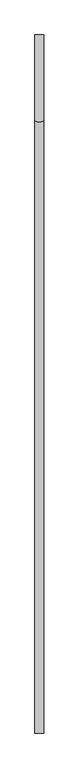
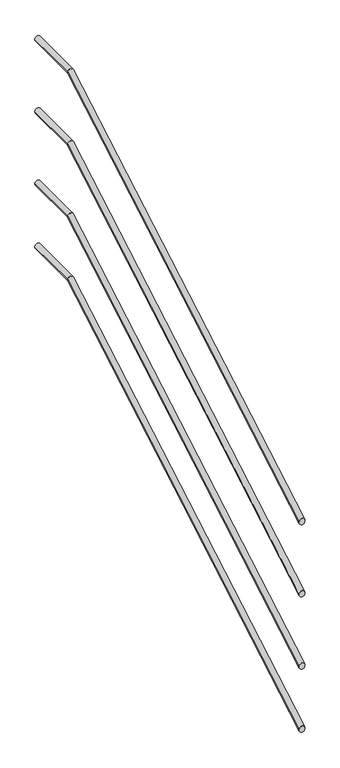
"""IFC4 building model written with IfcOpenShell, lengths in millimetres: railing geometry."""

from ifc_helpers import new_model, si_unit, frame, origin, place, context, project, spatial, circle_curve, ellipse_curve, source, transform, mapped, element, save
from ifc_brep_helpers import plane_surface, cylinder_surface, advanced_brep


def railing_984455d7(model_context):
    return source(origin(), model_context, "Body", "AdvancedBrep", [
        advanced_brep(
        [(-1890.4, 13399.5208589, 4296.7361432), (-1860.4, 13399.5208589, 4296.7361432), (-1890.4, 15503.5584173, 5517.9030398), (-1860.4, 15503.5584173, 5517.9030398), (-1890.4, 15799.5208589, 5517.9030398), (-1860.4, 15799.5208589, 5517.9030398)],
        [
            (0, 1, ellipse_curve(frame((-1875.4, 13399.5208589, 4296.7361432), z_axis=(0.0, -1.0, 0.0), x_axis=(0.0, 0.0, -1.0)), 17.3433672, 15.0)),
            (1, 0, ellipse_curve(frame((-1875.4, 13399.5208589, 4296.7361432), z_axis=(0.0, -1.0, 0.0), x_axis=(0.0, 0.0, -1.0)), 17.3433672, 15.0)),
            (0, 2),
            (2, 3, ellipse_curve(frame((-1875.4, 15503.5584173, 5517.9030398), z_axis=(0.0, -0.9656303515230847, -0.2599192648062162), x_axis=(0.0, 0.2599192648062171, -0.9656303515230844)), 15.5338945, 15.0)),
            (3, 1),
            (3, 2, ellipse_curve(frame((-1875.4, 15503.5584173, 5517.9030398), z_axis=(0.0, -0.9656303515230847, -0.2599192648062162), x_axis=(0.0, 0.2599192648062171, -0.9656303515230844)), 15.5338945, 15.0)),
            (4, 5, circle_curve(frame((-1875.4, 15799.5208589, 5517.9030398), z_axis=(0.0, 1.0, 0.0), x_axis=(1.0, 0.0, 0.0)), 15.0)),
            (5, 4, circle_curve(frame((-1875.4, 15799.5208589, 5517.9030398), z_axis=(0.0, 1.0, 0.0), x_axis=(1.0, 0.0, 0.0)), 15.0)),
            (2, 4),
            (5, 3),
        ],
        [
            plane_surface(frame((-1875.4, 13399.5208589, 4314.0795104), z_axis=(0.0, -1.0, 0.0), x_axis=(0.0, 0.0, 1.0))),
            cylinder_surface(frame((-1875.4, 13407.0504368, 4301.1062512), z_axis=(0.0, -0.8648839515651922, -0.5019718620848966), x_axis=(1.0, 0.0, 0.0)), 15.0),
            plane_surface(frame((-1875.4, 15799.5208589, 5532.9030398), z_axis=(0.0, 1.0, 0.0), x_axis=(0.0, 0.0, 1.0))),
            cylinder_surface(frame((-1875.4, 15499.5208589, 5517.9030398), z_axis=(0.0, -1.0, 0.0), x_axis=(1.0, 0.0, 0.0)), 15.0),
        ],
        [
            (0, [[1, 2]]),
            (1, [[-1, 3, 4, 5]]),
            (1, [[-2, -5, 6, -3]]),
            (2, [[7, 8]]),
            (3, [[-4, 9, -8, 10]]),
            (3, [[-6, -10, -7, -9]]),
        ],
    ),
        advanced_brep(
        [(-1890.4, 13399.5208589, 3496.7361432), (-1860.4, 13399.5208589, 3496.7361432), (-1890.4, 15503.5584173, 4717.9030398), (-1860.4, 15503.5584173, 4717.9030398), (-1890.4, 15799.5208589, 4717.9030398), (-1860.4, 15799.5208589, 4717.9030398)],
        [
            (0, 1, ellipse_curve(frame((-1875.4, 13399.5208589, 3496.7361432), z_axis=(0.0, -1.0, 0.0), x_axis=(0.0, 0.0, -1.0)), 17.3433672, 15.0)),
            (1, 0, ellipse_curve(frame((-1875.4, 13399.5208589, 3496.7361432), z_axis=(0.0, -1.0, 0.0), x_axis=(0.0, 0.0, -1.0)), 17.3433672, 15.0)),
            (0, 2),
            (2, 3, ellipse_curve(frame((-1875.4, 15503.5584173, 4717.9030398), z_axis=(0.0, -0.9656303515230847, -0.2599192648062162), x_axis=(0.0, 0.2599192648062171, -0.9656303515230844)), 15.5338945, 15.0)),
            (3, 1),
            (3, 2, ellipse_curve(frame((-1875.4, 15503.5584173, 4717.9030398), z_axis=(0.0, -0.9656303515230847, -0.2599192648062162), x_axis=(0.0, 0.2599192648062171, -0.9656303515230844)), 15.5338945, 15.0)),
            (4, 5, circle_curve(frame((-1875.4, 15799.5208589, 4717.9030398), z_axis=(0.0, 1.0, 0.0), x_axis=(1.0, 0.0, 0.0)), 15.0)),
            (5, 4, circle_curve(frame((-1875.4, 15799.5208589, 4717.9030398), z_axis=(0.0, 1.0, 0.0), x_axis=(1.0, 0.0, 0.0)), 15.0)),
            (2, 4),
            (5, 3),
        ],
        [
            plane_surface(frame((-1875.4, 13399.5208589, 3514.0795104), z_axis=(0.0, -1.0, 0.0), x_axis=(0.0, 0.0, 1.0))),
            cylinder_surface(frame((-1875.4, 13407.0504368, 3501.1062512), z_axis=(0.0, -0.8648839515651922, -0.5019718620848966), x_axis=(1.0, 0.0, 0.0)), 15.0),
            plane_surface(frame((-1875.4, 15799.5208589, 4732.9030398), z_axis=(0.0, 1.0, 0.0), x_axis=(0.0, 0.0, 1.0))),
            cylinder_surface(frame((-1875.4, 15499.5208589, 4717.9030398), z_axis=(0.0, -1.0, 0.0), x_axis=(1.0, 0.0, 0.0)), 15.0),
        ],
        [
            (0, [[1, 2]]),
            (1, [[-1, 3, 4, 5]]),
            (1, [[-2, -5, 6, -3]]),
            (2, [[7, 8]]),
            (3, [[-4, 9, -8, 10]]),
            (3, [[-6, -10, -7, -9]]),
        ],
    ),
        advanced_brep(
        [(-1890.4, 13399.5208589, 3896.7361432), (-1860.4, 13399.5208589, 3896.7361432), (-1890.4, 15503.5584173, 5117.9030398), (-1860.4, 15503.5584173, 5117.9030398), (-1890.4, 15799.5208589, 5117.9030398), (-1860.4, 15799.5208589, 5117.9030398)],
        [
            (0, 1, ellipse_curve(frame((-1875.4, 13399.5208589, 3896.7361432), z_axis=(0.0, -1.0, 0.0), x_axis=(0.0, 0.0, -1.0)), 17.3433672, 15.0)),
            (1, 0, ellipse_curve(frame((-1875.4, 13399.5208589, 3896.7361432), z_axis=(0.0, -1.0, 0.0), x_axis=(0.0, 0.0, -1.0)), 17.3433672, 15.0)),
            (0, 2),
            (2, 3, ellipse_curve(frame((-1875.4, 15503.5584173, 5117.9030398), z_axis=(0.0, -0.9656303515230847, -0.2599192648062162), x_axis=(0.0, 0.2599192648062171, -0.9656303515230844)), 15.5338945, 15.0)),
            (3, 1),
            (3, 2, ellipse_curve(frame((-1875.4, 15503.5584173, 5117.9030398), z_axis=(0.0, -0.9656303515230847, -0.2599192648062162), x_axis=(0.0, 0.2599192648062171, -0.9656303515230844)), 15.5338945, 15.0)),
            (4, 5, circle_curve(frame((-1875.4, 15799.5208589, 5117.9030398), z_axis=(0.0, 1.0, 0.0), x_axis=(1.0, 0.0, 0.0)), 15.0)),
            (5, 4, circle_curve(frame((-1875.4, 15799.5208589, 5117.9030398), z_axis=(0.0, 1.0, 0.0), x_axis=(1.0, 0.0, 0.0)), 15.0)),
            (2, 4),
            (5, 3),
        ],
        [
            plane_surface(frame((-1875.4, 13399.5208589, 3914.0795104), z_axis=(0.0, -1.0, 0.0), x_axis=(0.0, 0.0, 1.0))),
            cylinder_surface(frame((-1875.4, 13407.0504368, 3901.1062512), z_axis=(0.0, -0.8648839515651922, -0.5019718620848966), x_axis=(1.0, 0.0, 0.0)), 15.0),
            plane_surface(frame((-1875.4, 15799.5208589, 5132.9030398), z_axis=(0.0, 1.0, 0.0), x_axis=(0.0, 0.0, 1.0))),
            cylinder_surface(frame((-1875.4, 15499.5208589, 5117.9030398), z_axis=(0.0, -1.0, 0.0), x_axis=(1.0, 0.0, 0.0)), 15.0),
        ],
        [
            (0, [[1, 2]]),
            (1, [[-1, 3, 4, 5]]),
            (1, [[-2, -5, 6, -3]]),
            (2, [[7, 8]]),
            (3, [[-4, 9, -8, 10]]),
            (3, [[-6, -10, -7, -9]]),
        ],
    ),
        advanced_brep(
        [(-1890.4, 13399.5208589, 3146.7361432), (-1860.4, 13399.5208589, 3146.7361432), (-1890.4, 15503.5584173, 4367.9030398), (-1860.4, 15503.5584173, 4367.9030398), (-1890.4, 15799.5208589, 4367.9030398), (-1860.4, 15799.5208589, 4367.9030398)],
        [
            (0, 1, ellipse_curve(frame((-1875.4, 13399.5208589, 3146.7361432), z_axis=(0.0, -1.0, 0.0), x_axis=(0.0, 0.0, -1.0)), 17.3433672, 15.0)),
            (1, 0, ellipse_curve(frame((-1875.4, 13399.5208589, 3146.7361432), z_axis=(0.0, -1.0, 0.0), x_axis=(0.0, 0.0, -1.0)), 17.3433672, 15.0)),
            (0, 2),
            (2, 3, ellipse_curve(frame((-1875.4, 15503.5584173, 4367.9030398), z_axis=(0.0, -0.9656303515230847, -0.2599192648062162), x_axis=(0.0, 0.2599192648062171, -0.9656303515230844)), 15.5338945, 15.0)),
            (3, 1),
            (3, 2, ellipse_curve(frame((-1875.4, 15503.5584173, 4367.9030398), z_axis=(0.0, -0.9656303515230847, -0.2599192648062162), x_axis=(0.0, 0.2599192648062171, -0.9656303515230844)), 15.5338945, 15.0)),
            (4, 5, circle_curve(frame((-1875.4, 15799.5208589, 4367.9030398), z_axis=(0.0, 1.0, 0.0), x_axis=(1.0, 0.0, 0.0)), 15.0)),
            (5, 4, circle_curve(frame((-1875.4, 15799.5208589, 4367.9030398), z_axis=(0.0, 1.0, 0.0), x_axis=(1.0, 0.0, 0.0)), 15.0)),
            (2, 4),
            (5, 3),
        ],
        [
            plane_surface(frame((-1875.4, 13399.5208589, 3164.0795104), z_axis=(0.0, -1.0, 0.0), x_axis=(0.0, 0.0, 1.0))),
            cylinder_surface(frame((-1875.4, 13407.0504368, 3151.1062512), z_axis=(0.0, -0.8648839515651922, -0.5019718620848966), x_axis=(1.0, 0.0, 0.0)), 15.0),
            plane_surface(frame((-1875.4, 15799.5208589, 4382.9030398), z_axis=(0.0, 1.0, 0.0), x_axis=(0.0, 0.0, 1.0))),
            cylinder_surface(frame((-1875.4, 15499.5208589, 4367.9030398), z_axis=(0.0, -1.0, 0.0), x_axis=(1.0, 0.0, 0.0)), 15.0),
        ],
        [
            (0, [[1, 2]]),
            (1, [[-1, 3, 4, 5]]),
            (1, [[-2, -5, 6, -3]]),
            (2, [[7, 8]]),
            (3, [[-4, 9, -8, 10]]),
            (3, [[-6, -10, -7, -9]]),
        ],
    ),
    ])


if __name__ == "__main__":
    model = new_model("IFC4")
    model_context = context("Model", 3, world=origin())
    ifc_project = project(units=[si_unit("LENGTHUNIT", "METRE", prefix="MILLI")], contexts=[model_context])
    site = spatial("IfcSite", under=ifc_project)
    building = spatial("IfcBuilding", under=site)
    placement = place(None, origin())
    railing_shape = railing_984455d7(model_context)
    element("IfcRailing", 1, at=placement, inside=building, context=model_context, shape_type="MappedRepresentation", body=[
        mapped(railing_shape, transform((0.0, 0.0, 0.0), x_axis=(1.0, 0.0, 0.0), y_axis=(0.0, 1.0, 0.0), z_axis=(0.0, 0.0, 1.0))),
    ])
    save(model, "model.ifc")

# Revit data of these elements
# Project information
#   H_Seismic Condition = "A as per ASCE 7-10"
#   H_Soil Condition = "C as per ASCE 7-10"
#   H_Basic Wind Speed = "58.3m/s ASCE7-10"
#   Building Name = "2ND FLOOR PLAN"
#   H_DS Project Code = "FAASA2302"
#   H_Project Abbreviation = "SACE2"
#   H_Project Division = "화공"
#   H_Project Finish = "2027-03-05"
#   H_Project Location = "Jafurah, Saudi Arabia"
#   H_Project Start = "2024-01-03"
#   H_Project Type = "EPC"
#   H_Smart Code = "FAASA2302"
#   Project Issue Date = "Issue Date"
#   Project Status = "Project Status"
#   Client Name = "Owner"
#   Project Address = "Enter address here"
#   Project Name = "Project Name"
#   Project Number = "0001"
